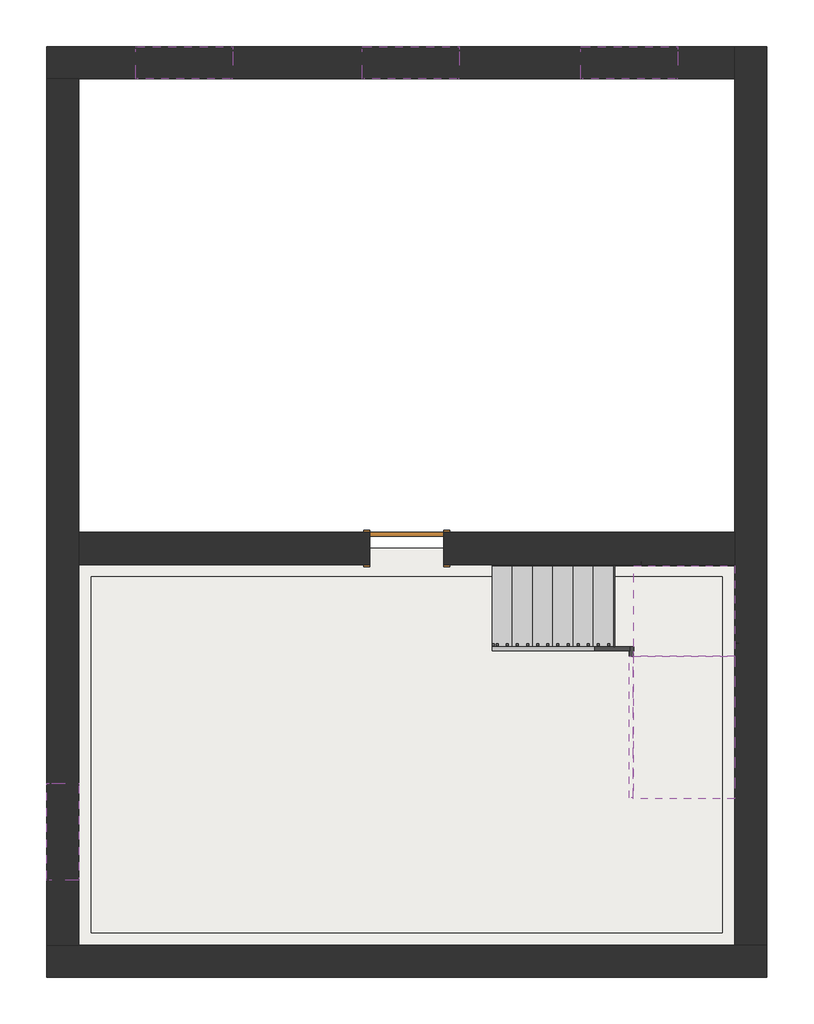
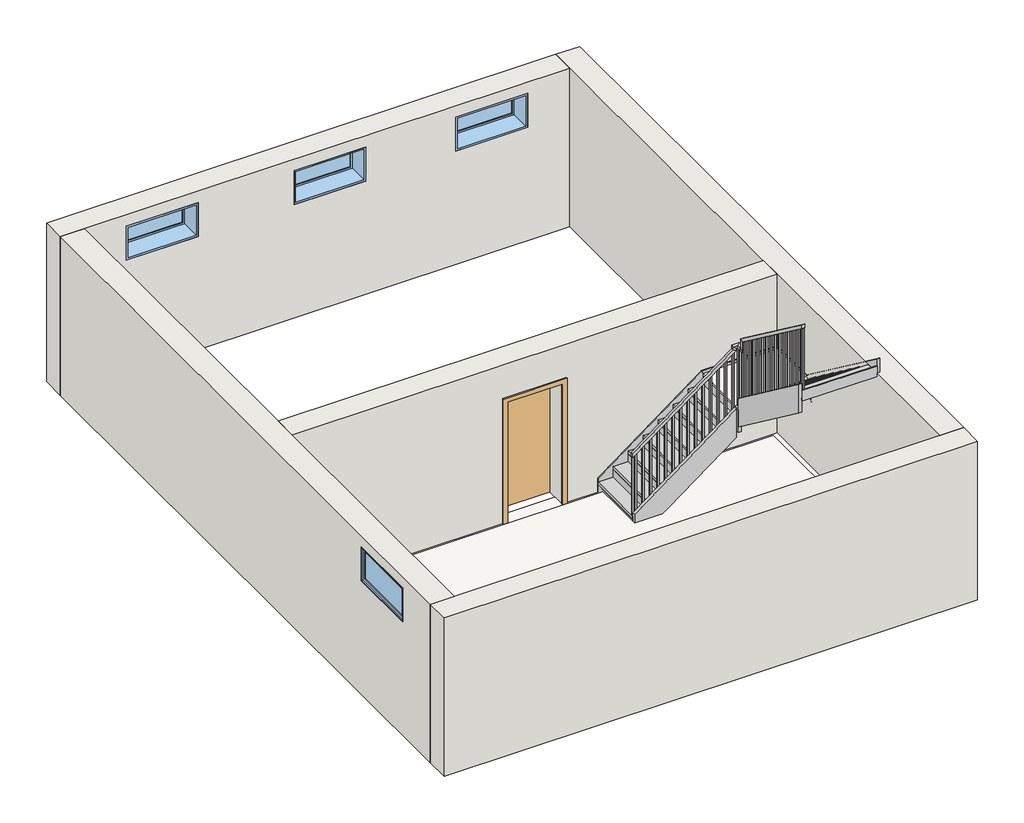
# One storey: 7 members, 5 walls, 4 windows, 3 slabs, 2 stair flights, 1 door, 1 railing.
"""IFC4 building model written with IfcOpenShell, lengths in millimetres."""

import ifcopenshell
import ifcopenshell.guid

model = None  # the IFC model being written
_history = None  # IfcOwnerHistory: only IFC2X3 demands one
_inside = {}  # id of a spatial element -> (the spatial element, [elements in it])
_under = {}  # id of a project, library or spatial element -> (it, [spatial elements below it])
_declared = {}  # id of a project -> (the project, [libraries it declares])
_typed = {}  # id of a type object -> (the type object, [elements of that type])
_made_of = {}  # id of a material, layer set ... -> (it, [elements and type objects made of it])


def new_model(schema):
    """Start an empty IFC model of exactly this schema.

    Asked for "IFC4X3", IfcOpenShell would pick the latest addendum, in which some entities
    have other attributes; the version numbers below select the first issue.
    IFC2X3 requires an IfcOwnerHistory on every rooted entity: one is made here for all.
    """
    global model, _history
    if schema == "IFC4X3":
        model = ifcopenshell.file(schema_version=(4, 3, 0, 0))
    else:
        model = ifcopenshell.file(schema=schema)
    _inside.clear()
    _under.clear()
    _declared.clear()
    _typed.clear()
    _made_of.clear()
    _history = None
    if model.schema == "IFC2X3":
        org = make("IfcOrganization", Name="unknown")
        user = make(
            "IfcPersonAndOrganization",
            ThePerson=make("IfcPerson", FamilyName="unknown"),
            TheOrganization=org,
        )
        app = make(
            "IfcApplication",
            ApplicationDeveloper=org,
            Version="unknown",
            ApplicationFullName="unknown",
            ApplicationIdentifier="unknown",
        )
        _history = make(
            "IfcOwnerHistory",
            OwningUser=user,
            OwningApplication=app,
            ChangeAction="ADDED",
            CreationDate=0,
        )
    return model


def make(cls, **values):
    """One entity of the class cls with the attributes given. An attribute that is None is left unset."""
    return model.create_entity(
        cls, **{name: value for name, value in values.items() if value is not None}
    )


def rooted(cls, **values):
    """An entity with a GlobalId (a new one), such as an element, a storey or a relation."""
    return make(cls, GlobalId=ifcopenshell.guid.new(), OwnerHistory=_history, **values)


def si_unit(unit_type, name, prefix=None):
    """IfcSIUnit, for example si_unit("LENGTHUNIT", "METRE", prefix="MILLI")."""
    return make("IfcSIUnit", UnitType=unit_type, Prefix=prefix, Name=name)


def assignment(units):
    """IfcUnitAssignment: the units of a project."""
    return None if units is None else make("IfcUnitAssignment", Units=units)


def point(xyz):
    """IfcCartesianPoint."""
    return None if xyz is None else make("IfcCartesianPoint", Coordinates=xyz)


def direction(xyz):
    """IfcDirection."""
    return None if xyz is None else make("IfcDirection", DirectionRatios=xyz)


def frame(location, z_axis=None, x_axis=None):
    """IfcAxis2Placement3D, a coordinate frame: its origin and axes. An axis left out is left unset."""
    return make(
        "IfcAxis2Placement3D",
        Location=point(location),
        Axis=direction(z_axis),
        RefDirection=direction(x_axis),
    )


def origin():
    """The frame at (0, 0, 0) with its axes left unset."""
    return frame((0.0, 0.0, 0.0))


def origin_with_axes():
    """The frame at (0, 0, 0) with the z axis (0, 0, 1) and the x axis (1, 0, 0) written out."""
    return frame((0.0, 0.0, 0.0), z_axis=(0.0, 0.0, 1.0), x_axis=(1.0, 0.0, 0.0))


def place(relative_to, where):
    """IfcLocalPlacement: puts the frame where relative to a parent placement (None: the world)."""
    return make(
        "IfcLocalPlacement", PlacementRelTo=relative_to, RelativePlacement=where
    )


def context(
    kind, dimensions, precision=None, world=None, true_north=None, identifier=None
):
    """IfcGeometricRepresentationContext, for example the 3D "Model" context."""
    return make(
        "IfcGeometricRepresentationContext",
        ContextIdentifier=identifier,
        ContextType=kind,
        CoordinateSpaceDimension=dimensions,
        Precision=precision,
        WorldCoordinateSystem=world,
        TrueNorth=true_north,
    )


def project(units=None, contexts=None):
    """IfcProject with its units and contexts."""
    return rooted(
        "IfcProject",
        Name="project",
        RepresentationContexts=contexts,
        UnitsInContext=assignment(units),
    )


def spatial(cls, under=None, at=None, **own):
    """A site, building, storey or space (cls), placed at a placement, below another one or the project."""
    s = rooted(cls, ObjectPlacement=at, **own)
    if under is not None:
        _under.setdefault(under.id(), (under, []))[1].append(s)
    return s


def polyline(points):
    """IfcPolyline through the points."""
    return make("IfcPolyline", Points=[point(p) for p in points])


def outline(outer, holes=None, kind="AREA"):
    """IfcArbitraryClosedProfileDef: a profile drawn as a closed curve; with holes, ...WithVoids."""
    if holes is None:
        return make("IfcArbitraryClosedProfileDef", ProfileType=kind, OuterCurve=outer)
    return make(
        "IfcArbitraryProfileDefWithVoids",
        ProfileType=kind,
        OuterCurve=outer,
        InnerCurves=holes,
    )


def extrude(swept, where, along, depth):
    """IfcExtrudedAreaSolid: the profile swept, set in the frame where, extruded along a direction by depth."""
    return make(
        "IfcExtrudedAreaSolid",
        SweptArea=swept,
        Position=where,
        ExtrudedDirection=direction(along),
        Depth=depth,
    )


def faces_of(points, faces, orient=None, outer=None):
    """IfcFace entities. A face is a list of loops; a loop is a list of indices into points, from 0.

    orient and outer hold one flag for each loop. By default every Orientation is true, the
    first loop of a face is its IfcFaceOuterBound and the others are IfcFaceBound.
    """
    made = []
    for i, loops in enumerate(faces):
        bounds = []
        for j, loop in enumerate(loops):
            is_outer = j == 0 if outer is None else outer[i][j]
            bounds.append(
                make(
                    "IfcFaceOuterBound" if is_outer else "IfcFaceBound",
                    Bound=make("IfcPolyLoop", Polygon=[points[k] for k in loop]),
                    Orientation=True if orient is None else orient[i][j],
                )
            )
        made.append(make("IfcFace", Bounds=bounds))
    return made


def faceted_brep(points, faces, orient=None, outer=None, voids=None):
    """IfcFacetedBrep: a solid bounded by flat faces; with voids (closed shells), ...WithVoids."""
    shared = [point(p) for p in points]
    hull = make("IfcClosedShell", CfsFaces=faces_of(shared, faces, orient, outer))
    if voids is None:
        return make("IfcFacetedBrep", Outer=hull)
    return make(
        "IfcFacetedBrepWithVoids",
        Outer=hull,
        Voids=[
            make(cls, CfsFaces=faces_of(shared, fs, o, b)) for cls, fs, o, b in voids
        ],
    )


def shape(context_of_items, identifier, shape_type, items):
    """IfcShapeRepresentation: the items that make up one representation, for example the "Body"."""
    return make(
        "IfcShapeRepresentation",
        ContextOfItems=context_of_items,
        RepresentationIdentifier=identifier,
        RepresentationType=shape_type,
        Items=items,
    )


def source(mapping_origin, context_of_items, identifier, shape_type, items):
    """IfcRepresentationMap: a shape defined once, which mapped items show again and again."""
    return make(
        "IfcRepresentationMap",
        MappingOrigin=mapping_origin,
        MappedRepresentation=shape(context_of_items, identifier, shape_type, items),
    )


def transform(
    local_origin,
    x_axis=None,
    y_axis=None,
    z_axis=None,
    scale=None,
    scale2=None,
    scale3=None,
    uniform=True,
):
    """IfcCartesianTransformationOperator3D, or its non-uniform kind. x_axis, y_axis, z_axis: its Axis1, 2, 3."""
    if uniform:
        return make(
            "IfcCartesianTransformationOperator3D",
            Axis1=direction(x_axis),
            Axis2=direction(y_axis),
            LocalOrigin=point(local_origin),
            Scale=scale,
            Axis3=direction(z_axis),
        )
    return make(
        "IfcCartesianTransformationOperator3DnonUniform",
        Axis1=direction(x_axis),
        Axis2=direction(y_axis),
        LocalOrigin=point(local_origin),
        Scale=scale,
        Axis3=direction(z_axis),
        Scale2=scale2,
        Scale3=scale3,
    )


def mapped(mapping_source, mapping_target):
    """IfcMappedItem: shows the shape of a source again, moved by a transform."""
    return make(
        "IfcMappedItem", MappingSource=mapping_source, MappingTarget=mapping_target
    )


def made_of(thing, what):
    """Note that an element or type object is made of a material, layer set ...; save() writes the relation."""
    if what is not None:
        _made_of.setdefault(what.id(), (what, []))[1].append(thing)
    return thing


def element(
    cls,
    number,
    at=None,
    inside=None,
    cuts=None,
    type_object=None,
    material=None,
    context=None,
    identifier="Body",
    shape_type=None,
    held_by="IfcProductDefinitionShape",
    body=None,
    shapes=None,
    **own,
):
    """One element of the class cls, such as IfcWall. Its Tag is "e" and its number.

    at: its placement. inside: the storey or other place that contains it. cuts: it is an
    opening in that element (IfcRelVoidsElement). A single representation is given by context,
    identifier, shape_type and body (its items); several are given by shapes. held_by: the class
    of the entity that holds the representations. save() writes the other relations.
    """
    e = rooted(cls, Tag="e%d" % number, ObjectPlacement=at, **own)
    if body is not None:
        shapes = [shape(context, identifier, shape_type, body)]
    if shapes is not None:
        e.Representation = make(held_by, Representations=shapes)
    if inside is not None:
        _inside.setdefault(inside.id(), (inside, []))[1].append(e)
    if cuts is not None:
        rooted(
            "IfcRelVoidsElement", RelatingBuildingElement=cuts, RelatedOpeningElement=e
        )
    if type_object is not None:
        _typed.setdefault(type_object.id(), (type_object, []))[1].append(e)
    return made_of(e, material)


def aggregate(whole, parts):
    """IfcRelAggregates: a whole, such as a stair, and the parts it consists of."""
    return rooted("IfcRelAggregates", RelatingObject=whole, RelatedObjects=parts)


def save(model, path):
    """Write the relations noted so far, then the file.

    IfcRelAggregates (storeys below a building ...), IfcRelContainedInSpatialStructure (elements
    in a storey), IfcRelDefinesByType, IfcRelAssociatesMaterial and IfcRelDeclares: one each for
    every whole, place, type object, material and project.
    """
    for whole, parts in _under.values():
        aggregate(whole, parts)
    for where, things in _inside.values():
        rooted(
            "IfcRelContainedInSpatialStructure",
            RelatedElements=things,
            RelatingStructure=where,
        )
    for kind, things in _typed.values():
        rooted("IfcRelDefinesByType", RelatedObjects=things, RelatingType=kind)
    for what, things in _made_of.values():
        rooted("IfcRelAssociatesMaterial", RelatedObjects=things, RelatingMaterial=what)
    for by, libraries in _declared.values():
        rooted("IfcRelDeclares", RelatingContext=by, RelatedDefinitions=libraries)
    model.write(path)


def door_d86ab3ce(model_context):
    return source(origin(), model_context, "Body", "SweptSolid", [
        extrude(outline(polyline([(2210.0, -533.5), (0.0, -533.5), (0.0, -457.5), (2134.0, -457.5), (2134.0, 457.5), (0.0, 457.5), (0.0, 533.5), (2210.0, 533.5), (2210.0, -533.5)])), frame((0.0, 200.0, 0.0), z_axis=(0.0, 1.0, 0.0), x_axis=(0.0, 0.0, 1.0)), (0.0, 0.0, 1.0), 25.0),
        extrude(outline(polyline([(2210.0, 533.5), (2210.0, -533.5), (0.0, -533.5), (0.0, -457.5), (2134.0, -457.5), (2134.0, 457.5), (0.0, 457.5), (0.0, 533.5), (2210.0, 533.5)])), frame((0.0, -225.0, 0.0), z_axis=(0.0, 1.0, 0.0), x_axis=(0.0, 0.0, 1.0)), (0.0, 0.0, 1.0), 25.0),
        extrude(outline(polyline([(457.5, 149.0), (-457.5, 149.0), (-457.5, 200.0), (457.5, 200.0), (457.5, 149.0)])), origin_with_axes(), (0.0, 0.0, 1.0), 2134.0),
    ])


def slab_18ee5c29(model_context):
    return source(origin(), model_context, "Body", "SweptSolid", [
        extrude(outline(polyline([(-11825.3533589, -8437.834784), (-10580.6631644, -8437.834784), (-10580.6631644, -9552.6519052), (-11830.6631644, -9552.6519052), (-11825.3533589, -9437.834784), (-11825.3533589, -8437.834784)])), frame((0.0, 0.0, 1443.3333333), z_axis=(0.0, 0.0, 1.0), x_axis=(1.0, 0.0, 0.0)), (0.0, 0.0, 1.0), 50.0),
    ])


def stair_flight_e7180eca(model_context):
    return source(origin(), model_context, "Body", "SweptSolid", [
        extrude(outline(polyline([(-13562.8533589, -9437.834784), (-13575.3533589, -9437.834784), (-13575.3533589, -8437.834784), (-13562.8533589, -8437.834784), (-13562.8533589, -9437.834784)])), origin_with_axes(), (0.0, 0.0, 1.0), 136.6666667),
        extrude(outline(polyline([(-13325.3533589, -8437.834784), (-13325.3533589, -9437.834784), (-13575.3533589, -9437.834784), (-13575.3533589, -8437.834784), (-13325.3533589, -8437.834784)])), frame((0.0, 0.0, 136.6666667), z_axis=(0.0, 0.0, 1.0), x_axis=(1.0, 0.0, 0.0)), (0.0, 0.0, 1.0), 50.0),
        extrude(outline(polyline([(-13312.8533589, -9437.834784), (-13325.3533589, -9437.834784), (-13325.3533589, -8437.834784), (-13312.8533589, -8437.834784), (-13312.8533589, -9437.834784)])), frame((0.0, 0.0, 136.6666667), z_axis=(0.0, 0.0, 1.0), x_axis=(1.0, 0.0, 0.0)), (0.0, 0.0, 1.0), 186.6666667),
        extrude(outline(polyline([(-13075.3533589, -8437.834784), (-13075.3533589, -9437.834784), (-13325.3533589, -9437.834784), (-13325.3533589, -8437.834784), (-13075.3533589, -8437.834784)])), frame((0.0, 0.0, 323.3333333), z_axis=(0.0, 0.0, 1.0), x_axis=(1.0, 0.0, 0.0)), (0.0, 0.0, 1.0), 50.0),
        extrude(outline(polyline([(-13062.8533589, -9437.834784), (-13075.3533589, -9437.834784), (-13075.3533589, -8437.834784), (-13062.8533589, -8437.834784), (-13062.8533589, -9437.834784)])), frame((0.0, 0.0, 323.3333333), z_axis=(0.0, 0.0, 1.0), x_axis=(1.0, 0.0, 0.0)), (0.0, 0.0, 1.0), 186.6666667),
        extrude(outline(polyline([(-12825.3533589, -8437.834784), (-12825.3533589, -9437.834784), (-13075.3533589, -9437.834784), (-13075.3533589, -8437.834784), (-12825.3533589, -8437.834784)])), frame((0.0, 0.0, 510.0), z_axis=(0.0, 0.0, 1.0), x_axis=(1.0, 0.0, 0.0)), (0.0, 0.0, 1.0), 50.0),
        extrude(outline(polyline([(-12812.8533589, -9437.834784), (-12825.3533589, -9437.834784), (-12825.3533589, -8437.834784), (-12812.8533589, -8437.834784), (-12812.8533589, -9437.834784)])), frame((0.0, 0.0, 510.0), z_axis=(0.0, 0.0, 1.0), x_axis=(1.0, 0.0, 0.0)), (0.0, 0.0, 1.0), 186.6666667),
        extrude(outline(polyline([(-12575.3533589, -8437.834784), (-12575.3533589, -9437.834784), (-12825.3533589, -9437.834784), (-12825.3533589, -8437.834784), (-12575.3533589, -8437.834784)])), frame((0.0, 0.0, 696.6666667), z_axis=(0.0, 0.0, 1.0), x_axis=(1.0, 0.0, 0.0)), (0.0, 0.0, 1.0), 50.0),
        extrude(outline(polyline([(-12562.8533589, -9437.834784), (-12575.3533589, -9437.834784), (-12575.3533589, -8437.834784), (-12562.8533589, -8437.834784), (-12562.8533589, -9437.834784)])), frame((0.0, 0.0, 696.6666667), z_axis=(0.0, 0.0, 1.0), x_axis=(1.0, 0.0, 0.0)), (0.0, 0.0, 1.0), 186.6666667),
        extrude(outline(polyline([(-12325.3533589, -8437.834784), (-12325.3533589, -9437.834784), (-12575.3533589, -9437.834784), (-12575.3533589, -8437.834784), (-12325.3533589, -8437.834784)])), frame((0.0, 0.0, 883.3333333), z_axis=(0.0, 0.0, 1.0), x_axis=(1.0, 0.0, 0.0)), (0.0, 0.0, 1.0), 50.0),
        extrude(outline(polyline([(-12312.8533589, -9437.834784), (-12325.3533589, -9437.834784), (-12325.3533589, -8437.834784), (-12312.8533589, -8437.834784), (-12312.8533589, -9437.834784)])), frame((0.0, 0.0, 883.3333333), z_axis=(0.0, 0.0, 1.0), x_axis=(1.0, 0.0, 0.0)), (0.0, 0.0, 1.0), 186.6666667),
        extrude(outline(polyline([(-12075.3533589, -8437.834784), (-12075.3533589, -9437.834784), (-12325.3533589, -9437.834784), (-12325.3533589, -8437.834784), (-12075.3533589, -8437.834784)])), frame((0.0, 0.0, 1070.0), z_axis=(0.0, 0.0, 1.0), x_axis=(1.0, 0.0, 0.0)), (0.0, 0.0, 1.0), 50.0),
        extrude(outline(polyline([(-12062.8533589, -9437.834784), (-12075.3533589, -9437.834784), (-12075.3533589, -8437.834784), (-12062.8533589, -8437.834784), (-12062.8533589, -9437.834784)])), frame((0.0, 0.0, 1070.0), z_axis=(0.0, 0.0, 1.0), x_axis=(1.0, 0.0, 0.0)), (0.0, 0.0, 1.0), 186.6666667),
        extrude(outline(polyline([(-11825.3533589, -8437.834784), (-11825.3533589, -9437.834784), (-12075.3533589, -9437.834784), (-12075.3533589, -8437.834784), (-11825.3533589, -8437.834784)])), frame((0.0, 0.0, 1256.6666667), z_axis=(0.0, 0.0, 1.0), x_axis=(1.0, 0.0, 0.0)), (0.0, 0.0, 1.0), 50.0),
        extrude(outline(polyline([(-11812.8533589, -9437.834784), (-11825.3533589, -9437.834784), (-11825.3533589, -8437.834784), (-11812.8533589, -8437.834784), (-11812.8533589, -9437.834784)])), frame((0.0, 0.0, 1256.6666667), z_axis=(0.0, 0.0, 1.0), x_axis=(1.0, 0.0, 0.0)), (0.0, 0.0, 1.0), 186.6666667),
    ])


def stair_flight_2d2a652e(model_context):
    return source(origin(), model_context, "Body", "SweptSolid", [
        extrude(outline(polyline([(-11830.6631644, -9565.1519052), (-11830.6631644, -9552.6519052), (-10580.6631644, -9552.6519052), (-10580.6631644, -9565.1519052), (-11830.6631644, -9565.1519052)])), frame((0.0, 0.0, 1443.3333333), z_axis=(0.0, 0.0, 1.0), x_axis=(1.0, 0.0, 0.0)), (0.0, 0.0, 1.0), 186.6666667),
        extrude(outline(polyline([(-10580.6631644, -9802.6519052), (-11830.6631644, -9802.6519052), (-11830.6631644, -9552.6519052), (-10580.6631644, -9552.6519052), (-10580.6631644, -9802.6519052)])), frame((0.0, 0.0, 1630.0), z_axis=(0.0, 0.0, 1.0), x_axis=(1.0, 0.0, 0.0)), (0.0, 0.0, 1.0), 50.0),
        extrude(outline(polyline([(-11830.6631644, -9815.1519052), (-11830.6631644, -9802.6519052), (-10580.6631644, -9802.6519052), (-10580.6631644, -9815.1519052), (-11830.6631644, -9815.1519052)])), frame((0.0, 0.0, 1630.0), z_axis=(0.0, 0.0, 1.0), x_axis=(1.0, 0.0, 0.0)), (0.0, 0.0, 1.0), 186.6666667),
        extrude(outline(polyline([(-10580.6631644, -10052.6519052), (-11830.6631644, -10052.6519052), (-11830.6631644, -9802.6519052), (-10580.6631644, -9802.6519052), (-10580.6631644, -10052.6519052)])), frame((0.0, 0.0, 1816.6666667), z_axis=(0.0, 0.0, 1.0), x_axis=(1.0, 0.0, 0.0)), (0.0, 0.0, 1.0), 50.0),
        extrude(outline(polyline([(-11830.6631644, -10065.1519052), (-11830.6631644, -10052.6519052), (-10580.6631644, -10052.6519052), (-10580.6631644, -10065.1519052), (-11830.6631644, -10065.1519052)])), frame((0.0, 0.0, 1816.6666667), z_axis=(0.0, 0.0, 1.0), x_axis=(1.0, 0.0, 0.0)), (0.0, 0.0, 1.0), 186.6666667),
        extrude(outline(polyline([(-10580.6631644, -10302.6519052), (-11830.6631644, -10302.6519052), (-11830.6631644, -10052.6519052), (-10580.6631644, -10052.6519052), (-10580.6631644, -10302.6519052)])), frame((0.0, 0.0, 2003.3333333), z_axis=(0.0, 0.0, 1.0), x_axis=(1.0, 0.0, 0.0)), (0.0, 0.0, 1.0), 50.0),
        extrude(outline(polyline([(-11830.6631644, -10315.1519052), (-11830.6631644, -10302.6519052), (-10580.6631644, -10302.6519052), (-10580.6631644, -10315.1519052), (-11830.6631644, -10315.1519052)])), frame((0.0, 0.0, 2003.3333333), z_axis=(0.0, 0.0, 1.0), x_axis=(1.0, 0.0, 0.0)), (0.0, 0.0, 1.0), 186.6666667),
        extrude(outline(polyline([(-10580.6631644, -10552.6519052), (-11830.6631644, -10552.6519052), (-11830.6631644, -10302.6519052), (-10580.6631644, -10302.6519052), (-10580.6631644, -10552.6519052)])), frame((0.0, 0.0, 2190.0), z_axis=(0.0, 0.0, 1.0), x_axis=(1.0, 0.0, 0.0)), (0.0, 0.0, 1.0), 50.0),
        extrude(outline(polyline([(-11830.6631644, -10565.1519052), (-11830.6631644, -10552.6519052), (-10580.6631644, -10552.6519052), (-10580.6631644, -10565.1519052), (-11830.6631644, -10565.1519052)])), frame((0.0, 0.0, 2190.0), z_axis=(0.0, 0.0, 1.0), x_axis=(1.0, 0.0, 0.0)), (0.0, 0.0, 1.0), 186.6666667),
        extrude(outline(polyline([(-10580.6631644, -10802.6519052), (-11830.6631644, -10802.6519052), (-11830.6631644, -10552.6519052), (-10580.6631644, -10552.6519052), (-10580.6631644, -10802.6519052)])), frame((0.0, 0.0, 2376.6666667), z_axis=(0.0, 0.0, 1.0), x_axis=(1.0, 0.0, 0.0)), (0.0, 0.0, 1.0), 50.0),
        extrude(outline(polyline([(-11830.6631644, -10815.1519052), (-11830.6631644, -10802.6519052), (-10580.6631644, -10802.6519052), (-10580.6631644, -10815.1519052), (-11830.6631644, -10815.1519052)])), frame((0.0, 0.0, 2376.6666667), z_axis=(0.0, 0.0, 1.0), x_axis=(1.0, 0.0, 0.0)), (0.0, 0.0, 1.0), 186.6666667),
        extrude(outline(polyline([(-10580.6631644, -11052.6519052), (-11830.6631644, -11052.6519052), (-11830.6631644, -10802.6519052), (-10580.6631644, -10802.6519052), (-10580.6631644, -11052.6519052)])), frame((0.0, 0.0, 2563.3333333), z_axis=(0.0, 0.0, 1.0), x_axis=(1.0, 0.0, 0.0)), (0.0, 0.0, 1.0), 50.0),
        extrude(outline(polyline([(-11830.6631644, -11065.1519052), (-11830.6631644, -11052.6519052), (-10580.6631644, -11052.6519052), (-10580.6631644, -11065.1519052), (-11830.6631644, -11065.1519052)])), frame((0.0, 0.0, 2563.3333333), z_axis=(0.0, 0.0, 1.0), x_axis=(1.0, 0.0, 0.0)), (0.0, 0.0, 1.0), 186.6666667),
        extrude(outline(polyline([(-11830.6631644, -11315.1519052), (-11830.6631644, -11302.6519052), (-10580.6631644, -11302.6519052), (-10580.6631644, -11315.1519052), (-11830.6631644, -11315.1519052)])), frame((0.0, 0.0, 2750.0), z_axis=(0.0, 0.0, 1.0), x_axis=(1.0, 0.0, 0.0)), (0.0, 0.0, 1.0), 186.6666667),
        extrude(outline(polyline([(-10580.6631644, -11302.6519052), (-11830.6631644, -11302.6519052), (-11830.6631644, -11052.6519052), (-10580.6631644, -11052.6519052), (-10580.6631644, -11302.6519052)])), frame((0.0, 0.0, 2750.0), z_axis=(0.0, 0.0, 1.0), x_axis=(1.0, 0.0, 0.0)), (0.0, 0.0, 1.0), 50.0),
    ])


def window_762fb1d9(model_context):
    return source(origin(), model_context, "Body", "SweptSolid", [
        extrude(outline(polyline([(-537.0, 178.0), (537.0, 178.0), (537.0, 166.0), (-537.0, 166.0), (-537.0, 178.0)])), frame((0.0, 0.0, 978.0), z_axis=(0.0, 0.0, 1.0), x_axis=(1.0, 0.0, 0.0)), (0.0, 0.0, 1.0), 474.0),
        extrude(outline(polyline([(1496.0, -581.0), (934.0, -581.0), (934.0, 581.0), (1496.0, 581.0), (1496.0, -581.0)]), holes=[polyline([(1452.0, -537.0), (1452.0, 537.0), (978.0, 537.0), (978.0, -537.0), (1452.0, -537.0)])]), frame((0.0, 150.0, 0.0), z_axis=(0.0, 1.0, 0.0), x_axis=(0.0, 0.0, 1.0)), (0.0, 0.0, 1.0), 44.0),
        extrude(outline(polyline([(1515.0, -600.0), (915.0, -600.0), (915.0, 600.0), (1515.0, 600.0), (1515.0, -600.0)]), holes=[polyline([(1496.0, -581.0), (1496.0, 581.0), (934.0, 581.0), (934.0, -581.0), (1496.0, -581.0)])]), frame((0.0, 150.0, 0.0), z_axis=(0.0, 1.0, 0.0), x_axis=(0.0, 0.0, 1.0)), (0.0, 0.0, 1.0), 63.0),
        extrude(outline(polyline([(1515.0, -600.0), (915.0, -600.0), (915.0, 600.0), (1515.0, 600.0), (1515.0, -600.0)]), holes=[polyline([(1483.0, -568.0), (1483.0, 568.0), (947.0, 568.0), (947.0, -568.0), (1483.0, -568.0)])]), frame((0.0, -187.0, 0.0), z_axis=(0.0, 1.0, 0.0), x_axis=(0.0, 0.0, 1.0)), (0.0, 0.0, 1.0), 337.0),
    ])


model = new_model("IFC4")

# Units and contexts
model_context = context("Model", 3, world=origin())
ifc_project = project(units=[si_unit("LENGTHUNIT", "METRE", prefix="MILLI")], contexts=[model_context])

# Site, building, storey
site = spatial("IfcSite", under=ifc_project)
building = spatial("IfcBuilding", under=site)
storey = spatial("IfcBuildingStorey", under=building, Name="Уровень 1", Elevation=0.0)

# Door
placement = place(None, origin())
door_shape = door_d86ab3ce(model_context)
element("IfcDoor", 1, ObjectType="Одиночные-Щитовые : 0915 x 2134 мм", at=placement, inside=storey, context=model_context, shape_type="MappedRepresentation", body=[
    mapped(door_shape, transform((-14630.6631644, -8222.3774925, 0.0), x_axis=(1.0, 0.0, 0.0), y_axis=(0.0, 1.0, 0.0), z_axis=(0.0, 0.0, 1.0))),
])

# Members
element("IfcMember", 2, ObjectType="Косоур/тетива - Ширина 50 мм", at=placement, inside=storey, context=model_context, shape_type="SweptSolid", body=[
    extrude(outline(polyline([(252.6673789, -13575.3533589), (0.0, -13575.3533589), (0.0, -13245.1742151), (1143.3333333, -11713.9242151), (1543.3333333, -11846.7828842), (252.6673789, -13575.3533589)])), frame((0.0, -8437.834784, 0.0), z_axis=(0.0, 1.0, 0.0), x_axis=(0.0, 0.0, 1.0)), (0.0, 0.0, 1.0), 50.0),
])
element("IfcMember", 3, ObjectType="Косоур/тетива - Ширина 50 мм", at=placement, inside=storey, context=model_context, shape_type="Brep", body=[
    faceted_brep([(-13575.3533589, -9487.834784, 0.0), (-13575.3533589, -9437.834784, 0.0), (-13245.1742151, -9437.834784, 0.0), (-13245.1742151, -9487.834784, 0.0), (-13575.3533589, -9487.834784, 252.6673789), (-13575.3533589, -9437.834784, 252.6673789), (-11877.7190853, -9487.834784, 1520.2343032), (-11875.4067971, -9437.834784, 1521.9608117), (-11875.4067971, -9437.834784, 1022.7596721), (-11877.7190853, -9487.834784, 1021.0331636)], [[[0, 1, 2, 3]], [[4, 5, 1, 0]], [[5, 4, 6, 7]], [[1, 5, 7, 8, 2]], [[4, 0, 3, 9, 6]], [[2, 8, 9, 3]], [[6, 9, 8, 7]]]),
])
element("IfcMember", 4, ObjectType="Косоур/тетива - Ширина 50 мм", at=placement, inside=storey, context=model_context, shape_type="SweptSolid", body=[
    extrude(outline(polyline([(-9281.2223799, 1543.3333333), (-9414.081049, 1143.3333333), (-11302.6519052, 2553.4662393), (-11302.6519052, 3052.6673789), (-9281.2223799, 1543.3333333)])), frame((-10580.6631644, 0.0, 0.0), z_axis=(1.0, 0.0, 0.0), x_axis=(0.0, 1.0, 0.0)), (0.0, 0.0, 1.0), 50.0),
])
element("IfcMember", 5, ObjectType="Косоур/тетива - Ширина 50 мм", at=placement, inside=storey, context=model_context, shape_type="SweptSolid", body=[
    extrude(outline(polyline([(-9552.6519052, 1746.0007122), (-9552.6519052, 1246.7995726), (-11302.6519052, 2553.4662393), (-11302.6519052, 3052.6673789), (-9552.6519052, 1746.0007122)])), frame((-11880.6631644, 0.0, 0.0), z_axis=(1.0, 0.0, 0.0), x_axis=(0.0, 1.0, 0.0)), (0.0, 0.0, 1.0), 50.0),
])
element("IfcMember", 6, ObjectType="Косоур/тетива - Ширина 50 мм", at=placement, inside=storey, context=model_context, shape_type="Brep", body=[
    faceted_brep([(-10580.6631644, -9281.2223799, 1543.3333333), (-10530.6631644, -9281.2223799, 1543.3333333), (-10530.6631644, -8387.834784, 1543.3333333), (-10580.6631644, -8437.834784, 1543.3333333), (-10580.6631644, -9414.081049, 1143.3333333), (-10580.6631644, -8437.834784, 1143.3333333), (-10530.6631644, -9414.081049, 1143.3333333), (-10530.6631644, -8387.834784, 1143.3333333)], [[[0, 1, 2, 3]], [[4, 0, 3, 5]], [[6, 4, 5, 7]], [[1, 6, 7, 2]], [[1, 0, 4, 6]], [[2, 7, 5, 3]]]),
])
element("IfcMember", 7, ObjectType="Косоур/тетива - Ширина 50 мм", at=placement, inside=storey, context=model_context, shape_type="Brep", body=[
    faceted_brep([(-10580.6631644, -8437.834784, 1543.3333333), (-10530.6631644, -8387.834784, 1543.3333333), (-11846.7828842, -8387.834784, 1543.3333333), (-11846.7828842, -8437.834784, 1543.3333333), (-10580.6631644, -8437.834784, 1143.3333333), (-11713.9242151, -8437.834784, 1143.3333333), (-10530.6631644, -8387.834784, 1143.3333333), (-11713.9242151, -8387.834784, 1143.3333333)], [[[0, 1, 2, 3]], [[4, 0, 3, 5]], [[6, 4, 5, 7]], [[1, 6, 7, 2]], [[1, 0, 4, 6]], [[2, 7, 5, 3]]]),
])
element("IfcMember", 8, ObjectType="Косоур/тетива - Ширина 50 мм", at=placement, inside=storey, context=model_context, shape_type="SweptSolid", body=[
    extrude(outline(polyline([(-11875.4067971, -9437.834784), (-11825.3533589, -9437.834784), (-11830.6631644, -9552.6519052), (-11880.7166026, -9552.6519052), (-11875.4067971, -9437.834784)])), frame((0.0, 0.0, 1143.3333333), z_axis=(0.0, 0.0, 1.0), x_axis=(1.0, 0.0, 0.0)), (0.0, 0.0, 1.0), 400.0),
])

# Railing
element("IfcRailing", 9, ObjectType="1100 мм", at=placement, inside=storey, context=model_context, shape_type="SolidModel", body=[
    faceted_brep([(-13575.3533589, -9387.434784, 1286.6666667), (-13575.3533589, -9387.434784, 1224.2665242), (-13575.3533589, -9437.434784, 1224.2665242), (-13575.3533589, -9437.434784, 1286.6666667), (-11898.7515698, -9387.434784, 2538.5293358), (-11848.7515698, -9387.434784, 2513.4625267), (-11848.7515698, -9437.434784, 2513.4625267), (-11898.7515698, -9437.434784, 2538.5293358), (-11779.1349452, -9529.4205131, 2593.3333333), (-11829.081564, -9527.1106936, 2593.3333333), (-11831.3913836, -9577.0573124, 2543.3333333), (-11781.4447647, -9579.367132, 2543.3333333), (-11778.3978995, -9513.4829315, 2543.3333333), (-11778.3978995, -9513.4829315, 2593.3333333), (-11828.3445184, -9511.1731119, 2543.3333333), (-11828.3445184, -9511.1731119, 2593.3333333), (-11898.7515698, -9387.434784, 2593.3333333), (-11848.7515698, -9387.434784, 2543.3333333), (-11848.7515698, -9437.434784, 2543.3333333), (-11898.7515698, -9437.434784, 2593.3333333), (-11772.5687066, -9387.434784, 2593.3333333), (-11772.5687066, -9387.434784, 2543.3333333), (-11824.934433, -9437.434784, 2543.3333333), (-11824.934433, -9437.434784, 2593.3333333)], [[[0, 1, 2, 3]], [[1, 0, 4, 5]], [[2, 1, 5, 6]], [[3, 2, 6, 7]], [[0, 3, 7, 4]], [[8, 9, 10, 11]], [[12, 13, 8, 11]], [[14, 12, 11, 10]], [[15, 14, 10, 9]], [[13, 15, 9, 8]], [[5, 4, 16, 17]], [[6, 5, 17, 18]], [[7, 6, 18, 19]], [[4, 7, 19, 16]], [[17, 16, 20, 21]], [[18, 17, 21, 22]], [[19, 18, 22, 23]], [[16, 19, 23, 20]], [[21, 20, 13, 12]], [[22, 21, 12, 14]], [[23, 22, 14, 15]], [[20, 23, 15, 13]]]),
    faceted_brep([(-11779.1349452, -9529.4205131, 2593.3333333), (-11781.4447647, -9579.367132, 2543.3333333), (-11831.3913836, -9577.0573124, 2543.3333333), (-11829.081564, -9527.1106936, 2593.3333333), (-11779.1349452, -9529.4205131, 2761.1792533), (-11829.081564, -9527.1106936, 2762.3372494), (-11831.3913836, -9577.0573124, 2737.2972022), (-11781.4447647, -9579.367132, 2736.1392061)], [[[0, 1, 2, 3]], [[4, 5, 6, 7]], [[1, 0, 4, 7]], [[2, 1, 7, 6]], [[3, 2, 6, 5]], [[0, 3, 5, 4]]]),
    faceted_brep([(-11780.2631644, -9528.2389128, 2761.7716323), (-11780.2631644, -9578.2389128, 2736.7048232), (-11830.2631644, -9578.2389128, 2736.7048232), (-11830.2631644, -9528.2389128, 2761.7716323), (-11780.2631644, -11302.6519052, 4086.6666667), (-11830.2631644, -11302.6519052, 4086.6666667), (-11830.2631644, -11302.6519052, 4024.2665242), (-11780.2631644, -11302.6519052, 4024.2665242)], [[[0, 1, 2, 3]], [[4, 5, 6, 7]], [[1, 0, 4, 7]], [[2, 1, 7, 6]], [[3, 2, 6, 5]], [[0, 3, 5, 4]]]),
    extrude(outline(polyline([(-11228.2389128, 3968.7048232), (-11228.2389128, 2800.0), (-11253.2389128, 2800.0), (-11253.2389128, 3987.3714898), (-11228.2389128, 3968.7048232)])), frame((-11817.7631644, 0.0, 0.0), z_axis=(1.0, 0.0, 0.0), x_axis=(0.0, 1.0, 0.0)), (0.0, 0.0, 1.0), 25.0),
    extrude(outline(polyline([(-11103.2389128, 3875.3714898), (-11103.2389128, 2800.0), (-11128.2389128, 2800.0), (-11128.2389128, 3894.0381565), (-11103.2389128, 3875.3714898)])), frame((-11817.7631644, 0.0, 0.0), z_axis=(1.0, 0.0, 0.0), x_axis=(0.0, 1.0, 0.0)), (0.0, 0.0, 1.0), 25.0),
    extrude(outline(polyline([(-10978.2389128, 3782.0381565), (-10978.2389128, 2613.3333333), (-11003.2389128, 2613.3333333), (-11003.2389128, 3800.7048232), (-10978.2389128, 3782.0381565)])), frame((-11817.7631644, 0.0, 0.0), z_axis=(1.0, 0.0, 0.0), x_axis=(0.0, 1.0, 0.0)), (0.0, 0.0, 1.0), 25.0),
    extrude(outline(polyline([(-10853.2389128, 3688.7048232), (-10853.2389128, 2613.3333333), (-10878.2389128, 2613.3333333), (-10878.2389128, 3707.3714898), (-10853.2389128, 3688.7048232)])), frame((-11817.7631644, 0.0, 0.0), z_axis=(1.0, 0.0, 0.0), x_axis=(0.0, 1.0, 0.0)), (0.0, 0.0, 1.0), 25.0),
    extrude(outline(polyline([(-10728.2389128, 3595.3714898), (-10728.2389128, 2426.6666667), (-10753.2389128, 2426.6666667), (-10753.2389128, 3614.0381565), (-10728.2389128, 3595.3714898)])), frame((-11817.7631644, 0.0, 0.0), z_axis=(1.0, 0.0, 0.0), x_axis=(0.0, 1.0, 0.0)), (0.0, 0.0, 1.0), 25.0),
    extrude(outline(polyline([(-10603.2389128, 3502.0381565), (-10603.2389128, 2426.6666667), (-10628.2389128, 2426.6666667), (-10628.2389128, 3520.7048232), (-10603.2389128, 3502.0381565)])), frame((-11817.7631644, 0.0, 0.0), z_axis=(1.0, 0.0, 0.0), x_axis=(0.0, 1.0, 0.0)), (0.0, 0.0, 1.0), 25.0),
    extrude(outline(polyline([(-10478.2389128, 3408.7048232), (-10478.2389128, 2240.0), (-10503.2389128, 2240.0), (-10503.2389128, 3427.3714898), (-10478.2389128, 3408.7048232)])), frame((-11817.7631644, 0.0, 0.0), z_axis=(1.0, 0.0, 0.0), x_axis=(0.0, 1.0, 0.0)), (0.0, 0.0, 1.0), 25.0),
    extrude(outline(polyline([(-10353.2389128, 3315.3714898), (-10353.2389128, 2240.0), (-10378.2389128, 2240.0), (-10378.2389128, 3334.0381565), (-10353.2389128, 3315.3714898)])), frame((-11817.7631644, 0.0, 0.0), z_axis=(1.0, 0.0, 0.0), x_axis=(0.0, 1.0, 0.0)), (0.0, 0.0, 1.0), 25.0),
    extrude(outline(polyline([(-10228.2389128, 3222.0381565), (-10228.2389128, 2053.3333333), (-10253.2389128, 2053.3333333), (-10253.2389128, 3240.7048232), (-10228.2389128, 3222.0381565)])), frame((-11817.7631644, 0.0, 0.0), z_axis=(1.0, 0.0, 0.0), x_axis=(0.0, 1.0, 0.0)), (0.0, 0.0, 1.0), 25.0),
    extrude(outline(polyline([(-10103.2389128, 3128.7048232), (-10103.2389128, 2053.3333333), (-10128.2389128, 2053.3333333), (-10128.2389128, 3147.3714898), (-10103.2389128, 3128.7048232)])), frame((-11817.7631644, 0.0, 0.0), z_axis=(1.0, 0.0, 0.0), x_axis=(0.0, 1.0, 0.0)), (0.0, 0.0, 1.0), 25.0),
    extrude(outline(polyline([(-9978.2389128, 3035.3714898), (-9978.2389128, 1866.6666667), (-10003.2389128, 1866.6666667), (-10003.2389128, 3054.0381565), (-9978.2389128, 3035.3714898)])), frame((-11817.7631644, 0.0, 0.0), z_axis=(1.0, 0.0, 0.0), x_axis=(0.0, 1.0, 0.0)), (0.0, 0.0, 1.0), 25.0),
    extrude(outline(polyline([(-9853.2389128, 2942.0381565), (-9853.2389128, 1866.6666667), (-9878.2389128, 1866.6666667), (-9878.2389128, 2960.7048232), (-9853.2389128, 2942.0381565)])), frame((-11817.7631644, 0.0, 0.0), z_axis=(1.0, 0.0, 0.0), x_axis=(0.0, 1.0, 0.0)), (0.0, 0.0, 1.0), 25.0),
    extrude(outline(polyline([(-9728.2389128, 2848.7048232), (-9728.2389128, 1680.0), (-9753.2389128, 1680.0), (-9753.2389128, 2867.3714898), (-9728.2389128, 2848.7048232)])), frame((-11817.7631644, 0.0, 0.0), z_axis=(1.0, 0.0, 0.0), x_axis=(0.0, 1.0, 0.0)), (0.0, 0.0, 1.0), 25.0),
    extrude(outline(polyline([(-9603.2389128, 2755.3714898), (-9603.2389128, 1680.0), (-9628.2389128, 1680.0), (-9628.2389128, 2774.0381565), (-9603.2389128, 2755.3714898)])), frame((-11817.7631644, 0.0, 0.0), z_axis=(1.0, 0.0, 0.0), x_axis=(0.0, 1.0, 0.0)), (0.0, 0.0, 1.0), 25.0),
    extrude(outline(polyline([(-11813.5480441, -9461.803948), (-11788.5747347, -9462.9588577), (-11789.7296445, -9487.9321672), (-11814.7029539, -9486.7772574), (-11813.5480441, -9461.803948)])), frame((0.0, 0.0, 1493.3333333), z_axis=(0.0, 0.0, 1.0), x_axis=(1.0, 0.0, 0.0)), (0.0, 0.0, 1.0), 1050.0),
    extrude(outline(polyline([(-11900.3533589, -9424.934784), (-11900.3533589, -9399.934784), (-11875.3533589, -9399.934784), (-11875.3533589, -9424.934784), (-11900.3533589, -9424.934784)])), frame((0.0, 0.0, 1306.6666667), z_axis=(0.0, 0.0, 1.0), x_axis=(1.0, 0.0, 0.0)), (0.0, 0.0, 1.0), 1236.6666667),
    extrude(outline(polyline([(2381.5998575, -12025.3533589), (1306.6666667, -12025.3533589), (1306.6666667, -12000.3533589), (2400.2665242, -12000.3533589), (2381.5998575, -12025.3533589)])), frame((0.0, -9424.934784, 0.0), z_axis=(0.0, 1.0, 0.0), x_axis=(0.0, 0.0, 1.0)), (0.0, 0.0, 1.0), 25.0),
    extrude(outline(polyline([(2288.2665242, -12150.3533589), (1120.0, -12150.3533589), (1120.0, -12125.3533589), (2306.9331909, -12125.3533589), (2288.2665242, -12150.3533589)])), frame((0.0, -9424.934784, 0.0), z_axis=(0.0, 1.0, 0.0), x_axis=(0.0, 0.0, 1.0)), (0.0, 0.0, 1.0), 25.0),
    extrude(outline(polyline([(2194.9331909, -12275.3533589), (1120.0, -12275.3533589), (1120.0, -12250.3533589), (2213.5998575, -12250.3533589), (2194.9331909, -12275.3533589)])), frame((0.0, -9424.934784, 0.0), z_axis=(0.0, 1.0, 0.0), x_axis=(0.0, 0.0, 1.0)), (0.0, 0.0, 1.0), 25.0),
    extrude(outline(polyline([(2101.5998575, -12400.3533589), (933.3333333, -12400.3533589), (933.3333333, -12375.3533589), (2120.2665242, -12375.3533589), (2101.5998575, -12400.3533589)])), frame((0.0, -9424.934784, 0.0), z_axis=(0.0, 1.0, 0.0), x_axis=(0.0, 0.0, 1.0)), (0.0, 0.0, 1.0), 25.0),
    extrude(outline(polyline([(2008.2665242, -12525.3533589), (933.3333333, -12525.3533589), (933.3333333, -12500.3533589), (2026.9331909, -12500.3533589), (2008.2665242, -12525.3533589)])), frame((0.0, -9424.934784, 0.0), z_axis=(0.0, 1.0, 0.0), x_axis=(0.0, 0.0, 1.0)), (0.0, 0.0, 1.0), 25.0),
    extrude(outline(polyline([(1914.9331909, -12650.3533589), (746.6666667, -12650.3533589), (746.6666667, -12625.3533589), (1933.5998575, -12625.3533589), (1914.9331909, -12650.3533589)])), frame((0.0, -9424.934784, 0.0), z_axis=(0.0, 1.0, 0.0), x_axis=(0.0, 0.0, 1.0)), (0.0, 0.0, 1.0), 25.0),
    extrude(outline(polyline([(1821.5998575, -12775.3533589), (746.6666667, -12775.3533589), (746.6666667, -12750.3533589), (1840.2665242, -12750.3533589), (1821.5998575, -12775.3533589)])), frame((0.0, -9424.934784, 0.0), z_axis=(0.0, 1.0, 0.0), x_axis=(0.0, 0.0, 1.0)), (0.0, 0.0, 1.0), 25.0),
    extrude(outline(polyline([(1728.2665242, -12900.3533589), (560.0, -12900.3533589), (560.0, -12875.3533589), (1746.9331909, -12875.3533589), (1728.2665242, -12900.3533589)])), frame((0.0, -9424.934784, 0.0), z_axis=(0.0, 1.0, 0.0), x_axis=(0.0, 0.0, 1.0)), (0.0, 0.0, 1.0), 25.0),
    extrude(outline(polyline([(1634.9331909, -13025.3533589), (560.0, -13025.3533589), (560.0, -13000.3533589), (1653.5998575, -13000.3533589), (1634.9331909, -13025.3533589)])), frame((0.0, -9424.934784, 0.0), z_axis=(0.0, 1.0, 0.0), x_axis=(0.0, 0.0, 1.0)), (0.0, 0.0, 1.0), 25.0),
    extrude(outline(polyline([(1541.5998575, -13150.3533589), (373.3333333, -13150.3533589), (373.3333333, -13125.3533589), (1560.2665242, -13125.3533589), (1541.5998575, -13150.3533589)])), frame((0.0, -9424.934784, 0.0), z_axis=(0.0, 1.0, 0.0), x_axis=(0.0, 0.0, 1.0)), (0.0, 0.0, 1.0), 25.0),
    extrude(outline(polyline([(1448.2665242, -13275.3533589), (373.3333333, -13275.3533589), (373.3333333, -13250.3533589), (1466.9331909, -13250.3533589), (1448.2665242, -13275.3533589)])), frame((0.0, -9424.934784, 0.0), z_axis=(0.0, 1.0, 0.0), x_axis=(0.0, 0.0, 1.0)), (0.0, 0.0, 1.0), 25.0),
    extrude(outline(polyline([(1354.9331909, -13400.3533589), (186.6666667, -13400.3533589), (186.6666667, -13375.3533589), (1373.5998575, -13375.3533589), (1354.9331909, -13400.3533589)])), frame((0.0, -9424.934784, 0.0), z_axis=(0.0, 1.0, 0.0), x_axis=(0.0, 0.0, 1.0)), (0.0, 0.0, 1.0), 25.0),
    extrude(outline(polyline([(1261.5998575, -13525.3533589), (186.6666667, -13525.3533589), (186.6666667, -13500.3533589), (1280.2665242, -13500.3533589), (1261.5998575, -13525.3533589)])), frame((0.0, -9424.934784, 0.0), z_axis=(0.0, 1.0, 0.0), x_axis=(0.0, 0.0, 1.0)), (0.0, 0.0, 1.0), 25.0),
    extrude(outline(polyline([(-11817.1723642, -9540.1748032), (-11792.1990548, -9541.3297129), (-11793.3539645, -9566.3030224), (-11818.327274, -9565.1481126), (-11817.1723642, -9540.1748032)])), frame((0.0, 0.0, 1493.3333333), z_axis=(0.0, 0.0, 1.0), x_axis=(1.0, 0.0, 0.0)), (0.0, 0.0, 1.0), 1050.0),
    extrude(outline(polyline([(-11811.2515698, -9424.934784), (-11811.2515698, -9399.934784), (-11786.2515698, -9399.934784), (-11786.2515698, -9424.934784), (-11811.2515698, -9424.934784)])), frame((0.0, 0.0, 1493.3333333), z_axis=(0.0, 0.0, 1.0), x_axis=(1.0, 0.0, 0.0)), (0.0, 0.0, 1.0), 1050.0),
    extrude(outline(polyline([(-11277.6519052, 4005.5998575), (-11277.6519052, 2800.0), (-11302.6519052, 2800.0), (-11302.6519052, 4024.2665242), (-11277.6519052, 4005.5998575)])), frame((-11817.7631644, 0.0, 0.0), z_axis=(1.0, 0.0, 0.0), x_axis=(0.0, 1.0, 0.0)), (0.0, 0.0, 1.0), 25.0),
    extrude(outline(polyline([(1224.2665242, -13575.3533589), (186.6666667, -13575.3533589), (186.6666667, -13550.3533589), (1242.9331909, -13550.3533589), (1224.2665242, -13575.3533589)])), frame((0.0, -9424.934784, 0.0), z_axis=(0.0, 1.0, 0.0), x_axis=(0.0, 0.0, 1.0)), (0.0, 0.0, 1.0), 25.0),
])

# Slabs
element("IfcSlab", 10, ObjectType="Бетон толщиной 160 мм с металлическим настилом толщиной 50 мм", at=placement, inside=storey, context=model_context, shape_type="SweptSolid", body=[
    extrude(outline(polyline([(-10380.6631644, -13122.3774925), (-18680.6631644, -13122.3774925), (-18680.6631644, -8222.3774925), (-10380.6631644, -8222.3774925), (-10380.6631644, -13122.3774925)])), frame((0.0, 0.0, -210.0), z_axis=(0.0, 0.0, 1.0), x_axis=(1.0, 0.0, 0.0)), (0.0, 0.0, 1.0), 210.0),
])
element("IfcSlab", 11, ObjectType="Бетон толщиной 160 мм с металлическим настилом толщиной 50 мм", at=placement, inside=storey, context=model_context, shape_type="SweptSolid", body=[
    extrude(outline(polyline([(-10730.6631644, -8572.3774925), (-10730.6631644, -12972.3774925), (-18530.6631644, -12972.3774925), (-18530.6631644, -8572.3774925), (-10730.6631644, -8572.3774925)])), frame((0.0, 0.0, -110.0), z_axis=(0.0, 0.0, 1.0), x_axis=(1.0, 0.0, 0.0)), (0.0, 0.0, 1.0), 210.0),
])
slab_shape = slab_18ee5c29(model_context)
element("IfcSlab", 12, ObjectType="Немонолитная площадка", at=placement, inside=storey, context=model_context, shape_type="MappedRepresentation", body=[
    mapped(slab_shape, transform((0.0, 0.0, 0.0), x_axis=(1.0, 0.0, 0.0), y_axis=(0.0, 1.0, 0.0), z_axis=(0.0, 0.0, 1.0))),
])

# Stair flights
stair_flight_shape = stair_flight_e7180eca(model_context)
element("IfcStairFlight", 13, ObjectType="Проступь 50 мм, подступенок 13 мм", at=placement, inside=storey, context=model_context, shape_type="MappedRepresentation", body=[
    mapped(stair_flight_shape, transform((0.0, 0.0, 0.0), x_axis=(1.0, 0.0, 0.0), y_axis=(0.0, 1.0, 0.0), z_axis=(0.0, 0.0, 1.0))),
])
stair_flight_2_shape = stair_flight_2d2a652e(model_context)
element("IfcStairFlight", 14, ObjectType="Проступь 50 мм, подступенок 13 мм", at=placement, inside=storey, context=model_context, shape_type="MappedRepresentation", body=[
    mapped(stair_flight_2_shape, transform((0.0, 0.0, 0.0), x_axis=(1.0, 0.0, 0.0), y_axis=(0.0, 1.0, 0.0), z_axis=(0.0, 0.0, 1.0))),
])

# Walls
element("IfcWall", 15, ObjectType="Фундамент - Бетон 400х2800", at=placement, inside=storey, context=model_context, shape_type="Brep", body=[
    faceted_brep([(-19080.6631644, -13522.3774925, 0.0), (-10180.6631644, -13522.3774925, 0.0), (-10180.6631644, -13522.3774925, 2800.0), (-19080.6631644, -13522.3774925, 2800.0), (-19080.6631644, -13122.3774925, 0.0), (-19080.6631644, -13122.3774925, 2800.0), (-18680.6631644, -13122.3774925, 2800.0), (-10580.6631644, -13122.3774925, 2800.0), (-10180.6631644, -13122.3774925, 2800.0), (-10180.6631644, -13122.3774925, 0.0), (-10580.6631644, -13122.3774925, 0.0), (-18680.6631644, -13122.3774925, 0.0)], [[[0, 1, 2, 3]], [[4, 5, 6, 7, 8, 9, 10, 11]], [[1, 0, 4, 11, 10, 9]], [[3, 2, 8, 7, 6, 5]], [[2, 1, 9, 8]], [[0, 3, 5, 4]]]),
])
element("IfcWall", 16, ObjectType="Фундамент - Бетон 400х2800", at=placement, inside=storey, context=model_context, shape_type="Brep", body=[
    faceted_brep([(-10180.6631644, -13122.3774925, 0.0), (-10180.6631644, -2022.3774925, 0.0), (-10180.6631644, -2022.3774925, 2800.0), (-10180.6631644, -13122.3774925, 2800.0), (-10580.6631644, -13122.3774925, 0.0), (-10580.6631644, -13122.3774925, 2800.0), (-10580.6631644, -8422.3774925, 2800.0), (-10580.6631644, -8022.3774925, 2800.0), (-10580.6631644, -2422.3774925, 2800.0), (-10580.6631644, -2022.3774925, 2800.0), (-10580.6631644, -2022.3774925, 0.0), (-10580.6631644, -2422.3774925, 0.0), (-10580.6631644, -8022.3774925, 0.0), (-10580.6631644, -8422.3774925, 0.0)], [[[0, 1, 2, 3]], [[4, 5, 6, 7, 8, 9, 10, 11, 12, 13]], [[1, 0, 4, 13, 12, 11, 10]], [[3, 2, 9, 8, 7, 6, 5]], [[0, 3, 5, 4]], [[2, 1, 10, 9]]]),
])
element("IfcWall", 17, ObjectType="Фундамент - Бетон 400х2800", at=placement, inside=storey, context=model_context, shape_type="Brep", body=[
    faceted_brep([(-10580.6631644, -2022.3774925, 0.0), (-19080.6631644, -2022.3774925, 0.0), (-19080.6631644, -2022.3774925, 2800.0), (-10580.6631644, -2022.3774925, 2800.0), (-12480.6631644, -2022.3774925, 2000.0), (-11280.6631644, -2022.3774925, 2000.0), (-11280.6631644, -2022.3774925, 2600.0), (-12480.6631644, -2022.3774925, 2600.0), (-15180.6631644, -2022.3774925, 2000.0), (-13980.6631644, -2022.3774925, 2000.0), (-13980.6631644, -2022.3774925, 2600.0), (-15180.6631644, -2022.3774925, 2600.0), (-17980.6631644, -2022.3774925, 2000.0), (-16780.6631644, -2022.3774925, 2000.0), (-16780.6631644, -2022.3774925, 2600.0), (-17980.6631644, -2022.3774925, 2600.0), (-10580.6631644, -2422.3774925, 0.0), (-10580.6631644, -2422.3774925, 2800.0), (-18680.6631644, -2422.3774925, 2800.0), (-19080.6631644, -2422.3774925, 2800.0), (-19080.6631644, -2422.3774925, 0.0), (-18680.6631644, -2422.3774925, 0.0), (-12480.6631644, -2422.3774925, 2000.0), (-12480.6631644, -2422.3774925, 2600.0), (-11280.6631644, -2422.3774925, 2600.0), (-11280.6631644, -2422.3774925, 2000.0), (-15180.6631644, -2422.3774925, 2000.0), (-15180.6631644, -2422.3774925, 2600.0), (-13980.6631644, -2422.3774925, 2600.0), (-13980.6631644, -2422.3774925, 2000.0), (-17980.6631644, -2422.3774925, 2000.0), (-17980.6631644, -2422.3774925, 2600.0), (-16780.6631644, -2422.3774925, 2600.0), (-16780.6631644, -2422.3774925, 2000.0)], [[[0, 1, 2, 3], [4, 5, 6, 7], [8, 9, 10, 11], [12, 13, 14, 15]], [[16, 17, 18, 19, 20, 21], [22, 23, 24, 25], [26, 27, 28, 29], [30, 31, 32, 33]], [[1, 0, 16, 21, 20]], [[3, 2, 19, 18, 17]], [[0, 3, 17, 16]], [[2, 1, 20, 19]], [[23, 22, 4, 7]], [[24, 23, 7, 6]], [[25, 24, 6, 5]], [[22, 25, 5, 4]], [[27, 26, 8, 11]], [[28, 27, 11, 10]], [[29, 28, 10, 9]], [[26, 29, 9, 8]], [[31, 30, 12, 15]], [[32, 31, 15, 14]], [[33, 32, 14, 13]], [[30, 33, 13, 12]]]),
])
element("IfcWall", 18, ObjectType="Фундамент - Бетон 400х2800", at=placement, inside=storey, context=model_context, shape_type="Brep", body=[
    faceted_brep([(-19080.6631644, -2422.3774925, 0.0), (-19080.6631644, -13122.3774925, 0.0), (-19080.6631644, -13122.3774925, 2800.0), (-19080.6631644, -2422.3774925, 2800.0), (-19080.6631644, -12322.3774925, 2000.0), (-19080.6631644, -11122.3774925, 2000.0), (-19080.6631644, -11122.3774925, 2600.0), (-19080.6631644, -12322.3774925, 2600.0), (-18680.6631644, -2422.3774925, 0.0), (-18680.6631644, -2422.3774925, 2800.0), (-18680.6631644, -8022.3774925, 2800.0), (-18680.6631644, -8422.3774925, 2800.0), (-18680.6631644, -13122.3774925, 2800.0), (-18680.6631644, -13122.3774925, 0.0), (-18680.6631644, -8422.3774925, 0.0), (-18680.6631644, -8022.3774925, 0.0), (-18680.6631644, -12322.3774925, 2000.0), (-18680.6631644, -12322.3774925, 2600.0), (-18680.6631644, -11122.3774925, 2600.0), (-18680.6631644, -11122.3774925, 2000.0)], [[[0, 1, 2, 3], [4, 5, 6, 7]], [[8, 9, 10, 11, 12, 13, 14, 15], [16, 17, 18, 19]], [[1, 0, 8, 15, 14, 13]], [[3, 2, 12, 11, 10, 9]], [[2, 1, 13, 12]], [[0, 3, 9, 8]], [[17, 16, 4, 7]], [[18, 17, 7, 6]], [[19, 18, 6, 5]], [[16, 19, 5, 4]]]),
])
element("IfcWall", 19, ObjectType="Фундамент - Бетон 400х2800", at=placement, inside=storey, context=model_context, shape_type="SweptSolid", body=[
    extrude(outline(polyline([(2134.0, -14173.1631644), (0.0, -14173.1631644), (0.0, -10580.6631644), (2800.0, -10580.6631644), (2800.0, -18680.6631644), (0.0, -18680.6631644), (0.0, -15088.1631644), (2134.0, -15088.1631644), (2134.0, -14173.1631644)])), frame((0.0, -8422.3774925, 0.0), z_axis=(0.0, 1.0, 0.0), x_axis=(0.0, 0.0, 1.0)), (0.0, 0.0, 1.0), 400.0),
])

# Windows
window_shape = window_762fb1d9(model_context)
element("IfcWindow", 20, ObjectType="Фиксированные : 1200х600", at=placement, inside=storey, context=model_context, shape_type="MappedRepresentation", body=[
    mapped(window_shape, transform((-18867.6631644, -11722.3774925, 1085.0), x_axis=(0.0, 1.0, 0.0), y_axis=(-1.0, 0.0, 0.0), z_axis=(0.0, 0.0, 1.0))),
])
element("IfcWindow", 21, ObjectType="Фиксированные : 1200х600", at=placement, inside=storey, context=model_context, shape_type="MappedRepresentation", body=[
    mapped(window_shape, transform((-11880.6631644, -2235.3774925, 1085.0), x_axis=(1.0, 0.0, 0.0), y_axis=(0.0, 1.0, 0.0), z_axis=(0.0, 0.0, 1.0))),
])
element("IfcWindow", 22, ObjectType="Фиксированные : 1200х600", at=placement, inside=storey, context=model_context, shape_type="MappedRepresentation", body=[
    mapped(window_shape, transform((-14580.6631644, -2235.3774925, 1085.0), x_axis=(1.0, 0.0, 0.0), y_axis=(0.0, 1.0, 0.0), z_axis=(0.0, 0.0, 1.0))),
])
element("IfcWindow", 23, ObjectType="Фиксированные : 1200х600", at=placement, inside=storey, context=model_context, shape_type="MappedRepresentation", body=[
    mapped(window_shape, transform((-17380.6631644, -2235.3774925, 1085.0), x_axis=(1.0, 0.0, 0.0), y_axis=(0.0, 1.0, 0.0), z_axis=(0.0, 0.0, 1.0))),
])

save(model, "model.ifc")

# Revit data of these elements
# Type "Одиночные-Щитовые : 0915 x 2134 мм"
#   Type Mark = "20"
#   Construction Type Id = "MDOOR"
#   Analytic Construction = "Металл"
#   Thickness = 51 mm
#   Heat Transfer Coefficient (U) = 3.7021 W/(m²·K)
#   Height = 2134 mm
#   Проекционная подчистка-соединение наруж. = 25 mm
#   Проекционная подчистка-соединение внутр. = 25 mm
#   Проекционное соединение по ширине = 76 mm
#   Width = 915 mm
#   Материал двери = Дверь - Панель
#   Материал каркаса = Дверь - Каркас
#   Visual Light Transmittance = 0
#   Solar Heat Gain Coefficient = 0
#   Function = (empty or 0)
#   Wall Closure = (empty or 0)
# Type "1100 мм"
#   built-in parameter 1008612 = 0.019685 (stored number, unit not read)
#   built-in parameter 1008611 = 0.019685 (stored number, unit not read)
#   built-in parameter 1008609 = 0.902231 (stored number, unit not read)
#   built-in parameter 1008604 = 0.19685 (stored number, unit not read)
#   built-in parameter 1008603 = 0.164042 (stored number, unit not read)
#   Railing Height = 1100 mm
#   built-in parameter 1008630 = 2
#   built-in parameter 1008610 = 2
#   built-in parameter 1008608 = 1
#   built-in parameter 1008618 = Балясина - Квадратная : 25  мм
# Type "Бетон толщиной 160 мм с металлическим настилом толщиной 50 мм"
#   Function = 0
#   Layers, outside or top first: 210 mm no material (function 1); 0 mm "Металлическая опалубка" (function 200)
# Type "Фундамент - Бетон 400х2800"
#   Layers, outside or top first: 400 mm "Бетон, монолитный" (function 1)
# Type "Фиксированные : 1200х600"
#   Type Mark = "19"
#   Construction Type Id = "GSP4R"
#   Analytic Construction = "Одинарное остекление стеклами Пилкингтон - 1/8 дюйма"
#   Visual Light Transmittance = 0.9
#   Solar Heat Gain Coefficient = 0.78
#   Heat Transfer Coefficient (U) = 3.6886 W/(m²·K)
#   Height = 600 mm
#   Высота подоконника по умолчанию = 915 mm
#   Width = 1200 mm
#   Вставка окна = 19 mm
#   Наружный материал каркаса = Переплет
#   Внутренний материал каркаса = Переплет
#   Материал оконного стекла = Стекло
#   Переплет = Переплет
#   Wall Closure = (empty or 0)
# Element 1 (IfcDoor, "Одиночные-Щитовые : 0915 x 2134 мм")
#   Phase Created = Новая конструкция
#   Materials on its faces: "Дверь - Каркас", "Дверь - Панель"
# Elements 2, 3, 4, 5, 6, 7, 8 (IfcMember, "Косоур/тетива - Ширина 50 мм")
#   Phase Created = Новая конструкция
# Element 9 (IfcRailing, "1100 мм")
#   Phase Created = Новая конструкция
# Element 10 (IfcSlab, "Бетон толщиной 160 мм с металлическим настилом толщиной 50 мм")
#   Height Offset From Level = 0 mm
#   built-in parameter 1001954 = 1
#   Phase Created = Новая конструкция
#   Materials on its faces: "Металлическая опалубка", "Этаж по умолчанию"
# Element 11 (IfcSlab, "Бетон толщиной 160 мм с металлическим настилом толщиной 50 мм")
#   Height Offset From Level = 100 mm
#   built-in parameter 1001954 = 1
#   Phase Created = Новая конструкция
#   Materials on its faces: "Металлическая опалубка", "Этаж по умолчанию"
# Element 12 (IfcSlab, "Немонолитная площадка")
#   Phase Created = Новая конструкция
# Elements 13, 14 (IfcStairFlight, "Проступь 50 мм, подступенок 13 мм")
#   Phase Created = Новая конструкция
# Elements 15, 16, 17, 18, 19 (IfcWall, "Фундамент - Бетон 400х2800")
#   Top Offset = 0 mm
#   Base Offset = 0 mm
#   wall height = 2800 mm
#   Phase Created = Новая конструкция
#   Base Constraint = Уровень 1
#   Top Constraint = Уровень 2
#   Materials on its faces: "Бетон, монолитный"
# Element 20 (IfcWindow, "Фиксированные : 1200х600")
#   Mark = "1"
#   Phase Created = Новая конструкция
#   Materials on its faces: "Переплет", "Стекло"
# Element 21 (IfcWindow, "Фиксированные : 1200х600")
#   Mark = "5"
#   Phase Created = Новая конструкция
#   Materials on its faces: "Переплет", "Стекло"
# Element 22 (IfcWindow, "Фиксированные : 1200х600")
#   Mark = "6"
#   Phase Created = Новая конструкция
#   Materials on its faces: "Переплет", "Стекло"
# Element 23 (IfcWindow, "Фиксированные : 1200х600")
#   Mark = "7"
#   Phase Created = Новая конструкция
#   Materials on its faces: "Переплет", "Стекло"
# Materials
#   "Дверь - Панель": class "Древесина", colour RGB 210 159 95, transparency 0, Cost = 0
#   "Дверь - Каркас": class "Разное", colour RGB 118 70 51, transparency 0, Cost = 0
#   "Металлическая опалубка": class "Металл", colour RGB 247 247 247, transparency 0, Description = "Сталь, прокатная отделка", Cost = 0
#   "Бетон, монолитный": class "Бетон", colour RGB 192 192 192, transparency 0, Description = "физический материал", Cost = 0
#   "Переплет": class "Древесина", colour RGB 224 178 126, transparency 0, Cost = 0
#   "Стекло": class "Стекло", colour RGB 0 128 192, transparency 0.9, Description = "Известково-натриевое стекло", Cost = 0
#   "Этаж по умолчанию": class "Разное", colour RGB 127 127 127, transparency 0, Cost = 0
